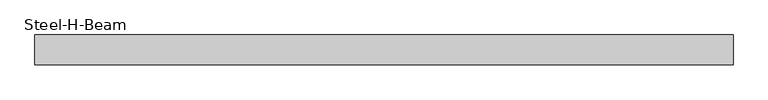
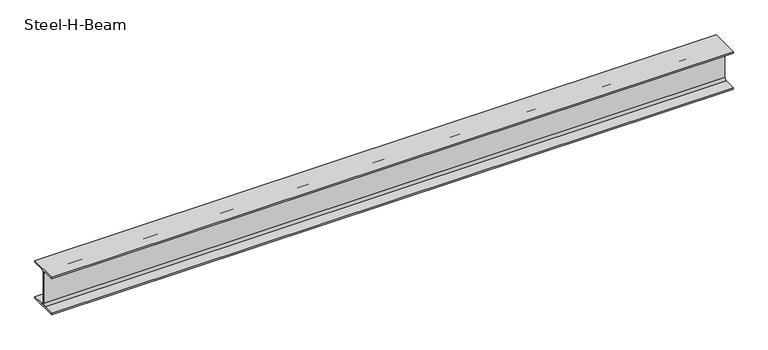
"""IFC4 building model written with IfcOpenShell, lengths in millimetres: beam geometry, Steel-H-Beam : BM121_H-340×250x9x14."""

from ifc_helpers import new_model, si_unit, point, frame, frame_2d, origin, place, context, project, spatial, polyline, circle_curve, trimmed, segment, composite_curve, outline, extrude, source, transform, mapped, element, save


def steel_h_beam_8a916b55(model_context):
    return source(origin(), model_context, "Body", "SweptSolid", [
        extrude(outline(composite_curve([segment(polyline([(125.0, -156.0), (125.0, -170.0), (-125.0, -170.0), (-125.0, -156.0), (-24.5, -156.0)]), True, "CONTINUOUS"), segment(trimmed(circle_curve(frame_2d((-24.5, -136.0)), 20.0), [point((-24.5, -156.0))], [point((-4.5, -136.0))], True, "CARTESIAN"), True, "CONTINUOUS"), segment(polyline([(-4.5, -136.0), (-4.5, 136.0)]), True, "CONTINUOUS"), segment(trimmed(circle_curve(frame_2d((-24.5, 136.0)), 20.0), [point((-4.5, 136.0))], [point((-24.5, 156.0))], True, "CARTESIAN"), True, "CONTINUOUS"), segment(polyline([(-24.5, 156.0), (-125.0, 156.0), (-125.0, 170.0), (125.0, 170.0), (125.0, 156.0), (24.5, 156.0)]), True, "CONTINUOUS"), segment(trimmed(circle_curve(frame_2d((24.5, 136.0)), 20.0), [point((24.5, 156.0))], [point((4.5, 136.0))], True, "CARTESIAN"), True, "CONTINUOUS"), segment(polyline([(4.5, 136.0), (4.5, -136.0)]), True, "CONTINUOUS"), segment(trimmed(circle_curve(frame_2d((24.5, -136.0)), 20.0), [point((4.5, -136.0))], [point((24.5, -156.0))], True, "CARTESIAN"), True, "CONTINUOUS"), segment(polyline([(24.5, -156.0), (125.0, -156.0)]), True, "CONTINUOUS")], self_intersect=False)), frame((-3014.9626863, 0.0, 0.0), z_axis=(1.0, 0.0, 0.0), x_axis=(0.0, 1.0, 0.0)), (0.0, 0.0, 1.0), 5826.388249),
    ])


if __name__ == "__main__":
    model = new_model("IFC4")
    model_context = context("Model", 3, world=origin())
    ifc_project = project(units=[si_unit("LENGTHUNIT", "METRE", prefix="MILLI")], contexts=[model_context])
    site = spatial("IfcSite", under=ifc_project)
    building = spatial("IfcBuilding", under=site)
    placement = place(None, origin())
    steel_h_beam_shape = steel_h_beam_8a916b55(model_context)
    element("IfcBeam", 1, ObjectType="Steel-H-Beam : BM121_H-340×250x9x14", at=placement, inside=building, context=model_context, shape_type="MappedRepresentation", body=[
        mapped(steel_h_beam_shape, transform((0.0, 0.0, 0.0), x_axis=(1.0, 0.0, 0.0), y_axis=(0.0, 1.0, 0.0), z_axis=(0.0, 0.0, 1.0))),
    ])
    save(model, "model.ifc")

# Revit data of these elements
# Type "Steel-H-Beam : BM121_H-340×250x9x14"
#   Surface Area = 1.62766 m²/m
#   Section Area = 101.514 cm²
#   Mass per Unit Length = 79.6882 kg/m
#   Length [instance default] = 3000 mm
#   B = 250 mm
#   H = 340 mm
#   r = 20 mm
#   tw = 9 mm
#   tf = 14 mm
#   hec_material4 [instance default] = none
#   hec_material3 [instance default] = none
#   hec_material2 [instance default] = none
#   hec_material1 [instance default] = none
#   Structural Material [instance default] = Steel, 45-345
#   Assembly Code = ""
# Element 1 (IfcBeam, "Steel-H-Beam : BM121_H-340×250x9x14")
#   hec_material4 = S01AA010-00002_Main Steel Structure Fabrication Work_Shelter/Building_Steel Painting/Coating_for Fireproofed Steel Surface, Surface Preparation & Primer Coat
#   hec_material3 = F01AC000-00002_Building/Shelter Fire Proofing Work_Intumescent Coating Type_1 hr. rating (UL 1709))
#   hec_material2 = S01AA010-00002_Main Steel Structure Fabrication Work_Shelter/Building_Steel Painting/Coating_for Fireproofed Steel Surface, Surface Preparation & Primer Coat
#   hec_material1 = S03AA028-00001_Main Steel Structure Erection Work_Shelter/Building_Medium Steel
#   Structural Material = S01AA002-00001_Main Steel Structure Fabrication Work_Shelter/Building_Medium Steel - Standard
#   Materials on its faces: "S01AA002-00001_Main Steel Structure Fabrication Work_Shelter/Building_Medium Steel - Standard"
# Materials
#   "Steel, 45-345": class "Metal", colour RGB 189 187 185, transparency 0, Description = "Steel 345 MPa", Cost = 0
#   "S01AA002-00001_Main Steel Structure Fabrication Work_Shelter/Building_Medium Steel - Standard": class "Metal", colour RGB 120 120 120, transparency 0, Comments = "(90KG/M>Weight≥30KG/M)", Description = "Structural steel 50ksi", W00) Work Master Code = "S01AA002-0001", W01) Work Master_Lv1 = "Main Steel Structure Fabrication Work", W02) Work Master_Lv2 = "Shelter/Building", W03) Work Master_Spec.1 = "Medium Steel - Standard (90KG/M>Weight≥30KG/M)", Cost = 0
#   "S01AA010-00002_Main Steel Structure Fabrication Work_Shelter/Building_Steel Painting/Coating_for Fireproofed Steel Surface, Surface Preparation & Primer Coat": class "Metal", colour RGB 120 120 120, transparency 0, Description = "Paint finished steel", W00) Work Master Code = "SS01AA010-00002", W01) Work Master_Lv1 = "Main Steel Structure Fabrication Work", W02) Work Master_Lv2 = "Shelter/Building", W03) Work Master_Spec.1 = "Steel Painting/Coating", W04) Work Master_Spec.2 = "for Fireproofed Steel Surface, Surface Preparation & Primer Coat", Cost = 0
#   "F01AC000-00002_Building/Shelter Fire Proofing Work_Intumescent Coating Type_1 hr. rating (UL 1709))": class "Metal", colour RGB 255 128 128, transparency 0, Description = "Paint finished steel", W00) Work Master Code = "F01AC000-00002", W01) Work Master_Lv1 = "Building/Shelter Fire Proofing Work", W02) Work Master_Lv2 = "Intumescent Coating Type", W03) Work Master_Spec.1 = "1 hr. rating (UL 1709)", Cost = 0
#   "S03AA028-00001_Main Steel Structure Erection Work_Shelter/Building_Medium Steel": class "Metal", colour RGB 120 120 120, transparency 0, Comments = "(90KG/M>Weight≥30KG/M)", Description = "Structural steel 50ksi", W00) Work Master Code = "S03AA028-0001", W01) Work Master_Lv1 = "Main Steel Structure Erection Work", W02) Work Master_Lv2 = "Shelter/Building", W03) Work Master_Spec.1 = "Medium Steel (90KG/M>Weight≥30KG/M)", Cost = 0
